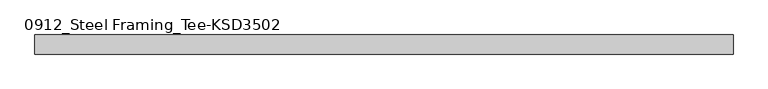
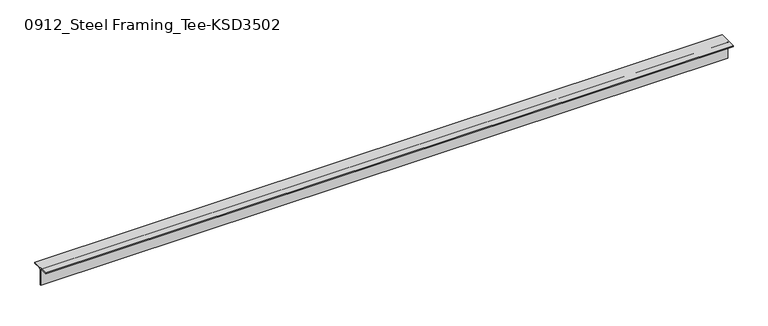
"""IFC4 building model written with IfcOpenShell, lengths in millimetres: member geometry, 0912_Steel Framing_Tee-KSD3502 : H_SB_ASB_CT-150x150x6.5x9."""

from ifc_helpers import new_model, si_unit, point, frame, frame_2d, origin, place, context, project, spatial, polyline, circle_curve, trimmed, segment, composite_curve, outline, extrude, source, transform, mapped, element, save


def member_0912_steel_framing_tee_ksd3502_945bf0ef(model_context):
    return source(origin(), model_context, "Body", "SweptSolid", [
        extrude(outline(composite_curve([segment(polyline([(-75.0, 75.0), (75.0, 75.0), (75.0, 66.0), (16.25, 66.0)]), True, "CONTINUOUS"), segment(trimmed(circle_curve(frame_2d((16.25, 53.0)), 13.0), [point((16.25, 66.0))], [point((3.25, 53.0))], True, "CARTESIAN"), True, "CONTINUOUS"), segment(polyline([(3.25, 53.0), (3.25, -75.0), (-3.25, -75.0), (-3.25, 53.0)]), True, "CONTINUOUS"), segment(trimmed(circle_curve(frame_2d((-16.25, 53.0)), 13.0), [point((-3.25, 53.0))], [point((-16.25, 66.0))], True, "CARTESIAN"), True, "CONTINUOUS"), segment(polyline([(-16.25, 66.0), (-75.0, 66.0), (-75.0, 75.0)]), True, "CONTINUOUS")], self_intersect=False)), frame((-2752.4, 0.0, 0.0), z_axis=(1.0, 0.0, 0.0), x_axis=(0.0, 1.0, 0.0)), (0.0, 0.0, 1.0), 5477.7),
    ])


if __name__ == "__main__":
    model = new_model("IFC4")
    model_context = context("Model", 3, world=origin())
    ifc_project = project(units=[si_unit("LENGTHUNIT", "METRE", prefix="MILLI")], contexts=[model_context])
    site = spatial("IfcSite", under=ifc_project)
    building = spatial("IfcBuilding", under=site)
    placement = place(None, origin())
    member_0912_steel_framing_tee_ksd3502_shape = member_0912_steel_framing_tee_ksd3502_945bf0ef(model_context)
    element("IfcMember", 1, ObjectType="0912_Steel Framing_Tee-KSD3502 : H_SB_ASB_CT-150x150x6.5x9", at=placement, inside=building, context=model_context, shape_type="MappedRepresentation", body=[
        mapped(member_0912_steel_framing_tee_ksd3502_shape, transform((0.0, 0.0, 0.0), x_axis=(1.0, 0.0, 0.0), y_axis=(0.0, 1.0, 0.0), z_axis=(0.0, 0.0, 1.0))),
    ])
    save(model, "model.ifc")

# Revit data of these elements
# Type "0912_Steel Framing_Tee-KSD3502 : H_SB_ASB_CT-150x150x6.5x9"
#   H_WM Code_1 = "S01AA003-00001 | Main Steel Structure Fabrication Work | Shelter/Building | Light Steel - Standard (30KG/M>Weight) | Material: (   )"
#   H_WM Code_2 = "S03AA029-00001 | Main Steel Structure Erection Work | Shelter/Building | Light Steel (30KG/M>Weight) | Material: (   )"
#   H_WM Code_3 = "S01AA010-00001 | Main Steel Structure Fabrication Work | Shelter/Building | Steel Painting/Coating | for Non-Fireproofed Steel Surface, Surface Preparation, Primer, Second & Final Coat | Material: (   )"
#   H_Q'ty Cal Type Tag = "SB-Q2"
#   Width = 15.0 cm
#   Web Thickness = 0.65 cm
#   Web Fillet = 1.3 cm
#   Section Area = 23.39 cm²
#   Perimeter = 0.60 m²/m
#   Nominal Weight = 18.40 kgf/m
#   Height = 15.0 cm
#   Flange Thickness = 0.9 cm
#   Centroid Vertical = 7.5 cm
#   Centroid Horizontal = 7.5 cm
#   Length [instance default] = 1.5000 m
#   Structural Material [instance default] = Steel, 45-345
#   Warping Constant = (empty or 0)
#   Torsional Moment of Inertia = 0
#   Section Name Key = ""
#   Plastic Modulus weak axis = 0
#   Plastic Modulus strong axis = 0
#   Moment of Inertia weak axis = 0
#   Moment of Inertia strong axis = 0
#   Elastic Modulus weak axis = 0
#   Elastic Modulus strong axis = 0
#   Bolt Spacing = 0
#   Assembly Code = ""
# Element 1 (IfcMember, "0912_Steel Framing_Tee-KSD3502 : H_SB_ASB_CT-150x150x6.5x9")
#   Structural Material = none
# Materials
#   "Steel, 45-345": class "Metal", colour RGB 189 187 185, transparency 0, Description = "Steel 345 MPa", Cost = 0
